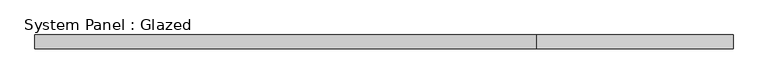
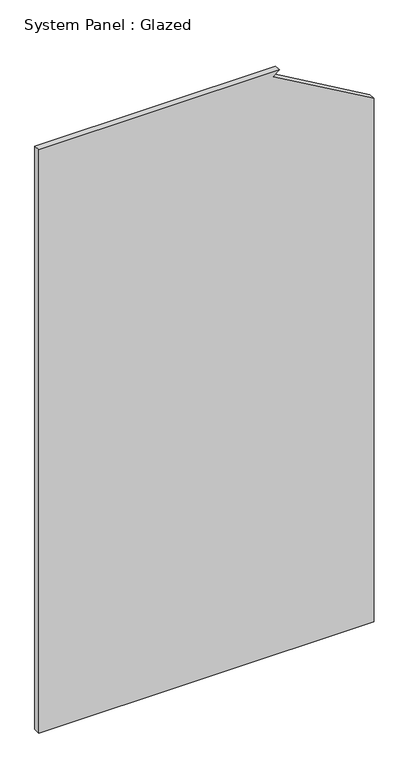
"""IFC4 building model written with IfcOpenShell, lengths in millimetres: plate geometry, System Panel : Glazed."""

from ifc_helpers import new_model, si_unit, frame, origin, place, context, project, spatial, polyline, outline, extrude, source, transform, mapped, element, save


def system_panel_glazed_2c07ae1a(model_context):
    return source(origin(), model_context, "Body", "SweptSolid", [
        extrude(outline(polyline([(0.0, -639.2857142), (0.0, 639.2857142), (2109.1765467, 639.2857142), (2331.6987298, 253.8659873), (2350.0, 278.8659873), (2350.0, -639.2857142), (0.0, -639.2857142)])), frame((0.0, 24.5, 0.0), z_axis=(0.0, 1.0, 0.0), x_axis=(0.0, 0.0, 1.0)), (0.0, 0.0, 1.0), 25.0),
    ])


if __name__ == "__main__":
    model = new_model("IFC4")
    model_context = context("Model", 3, world=origin())
    ifc_project = project(units=[si_unit("LENGTHUNIT", "METRE", prefix="MILLI")], contexts=[model_context])
    site = spatial("IfcSite", under=ifc_project)
    building = spatial("IfcBuilding", under=site)
    placement = place(None, origin())
    system_panel_glazed_shape = system_panel_glazed_2c07ae1a(model_context)
    element("IfcPlate", 1, ObjectType="System Panel : Glazed", at=placement, inside=building, context=model_context, shape_type="MappedRepresentation", body=[
        mapped(system_panel_glazed_shape, transform((0.0, 0.0, 0.0), x_axis=(1.0, 0.0, 0.0), y_axis=(0.0, 1.0, 0.0), z_axis=(0.0, 0.0, 1.0))),
    ])
    save(model, "model.ifc")

# Revit data of these elements
# Type "System Panel : Glazed"
#   Construction Type Id = "GSP4R"
#   Analytic Construction = "1/8 in Pilkington single glazing"
#   Visual Light Transmittance = 0.9
#   Solar Heat Gain Coefficient = 0.86
#   Heat Transfer Coefficient (U) = 6.7069 W/(m²·K)
#   Define Thermal Properties by = 1
# Element 1 (IfcPlate, "System Panel : Glazed")
#   Materials on its faces: "Glass"
# Materials
#   "Glass": class "Glass", colour RGB 0 128 192, transparency 0.75, Description = "Soda Lime Glass", Cost = 0
